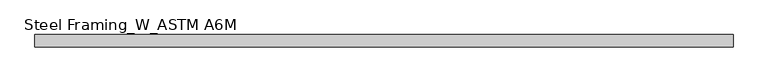
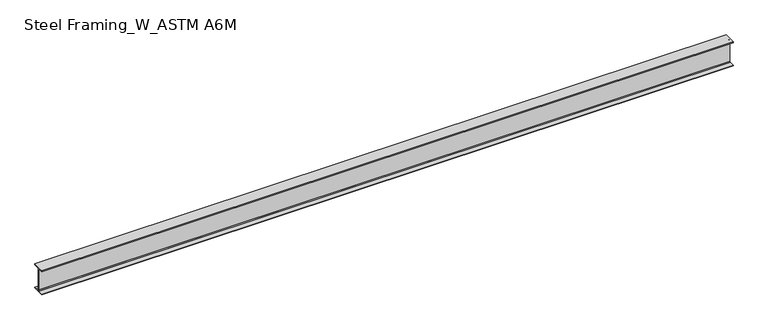
"""IFC4 building model written with IfcOpenShell, lengths in millimetres: beam geometry, Steel Framing_W_ASTM A6M : H_SB_AR_S02_W360x51_B4."""

from ifc_helpers import new_model, si_unit, point, frame, frame_2d, origin, place, context, project, spatial, polyline, circle_curve, trimmed, segment, composite_curve, outline, extrude, source, transform, mapped, element, save


def steel_framing_w_astm_a6m_aee8f6e1(model_context):
    return source(origin(), model_context, "Body", "SweptSolid", [
        extrude(outline(composite_curve([segment(polyline([(85.5, -166.4), (85.5, -178.0), (-85.5, -178.0), (-85.5, -166.4), (-13.72, -166.4)]), True, "CONTINUOUS"), segment(trimmed(circle_curve(frame_2d((-13.72, -156.3)), 10.1), [point((-13.72, -166.4))], [point((-3.62, -156.3))], True, "CARTESIAN"), True, "CONTINUOUS"), segment(polyline([(-3.62, -156.3), (-3.62, 156.3)]), True, "CONTINUOUS"), segment(trimmed(circle_curve(frame_2d((-13.72, 156.3)), 10.1), [point((-3.62, 156.3))], [point((-13.72, 166.4))], True, "CARTESIAN"), True, "CONTINUOUS"), segment(polyline([(-13.72, 166.4), (-85.5, 166.4), (-85.5, 178.0), (85.5, 178.0), (85.5, 166.4), (13.72, 166.4)]), True, "CONTINUOUS"), segment(trimmed(circle_curve(frame_2d((13.72, 156.3)), 10.1), [point((13.72, 166.4))], [point((3.62, 156.3))], True, "CARTESIAN"), True, "CONTINUOUS"), segment(polyline([(3.62, 156.3), (3.62, -156.3)]), True, "CONTINUOUS"), segment(trimmed(circle_curve(frame_2d((13.72, -156.3)), 10.1), [point((3.62, -156.3))], [point((13.72, -166.4))], True, "CARTESIAN"), True, "CONTINUOUS"), segment(polyline([(13.72, -166.4), (85.5, -166.4)]), True, "CONTINUOUS")], self_intersect=False)), frame((-4846.3, 0.0, 0.0), z_axis=(1.0, 0.0, 0.0), x_axis=(0.0, 1.0, 0.0)), (0.0, 0.0, 1.0), 9692.6),
    ])


if __name__ == "__main__":
    model = new_model("IFC4")
    model_context = context("Model", 3, world=origin())
    ifc_project = project(units=[si_unit("LENGTHUNIT", "METRE", prefix="MILLI")], contexts=[model_context])
    site = spatial("IfcSite", under=ifc_project)
    building = spatial("IfcBuilding", under=site)
    placement = place(None, origin())
    steel_framing_w_astm_a6m_shape = steel_framing_w_astm_a6m_aee8f6e1(model_context)
    element("IfcBeam", 1, ObjectType="Steel Framing_W_ASTM A6M : H_SB_AR_S02_W360x51_B4", at=placement, inside=building, context=model_context, shape_type="MappedRepresentation", body=[
        mapped(steel_framing_w_astm_a6m_shape, transform((0.0, 0.0, 0.0), x_axis=(1.0, 0.0, 0.0), y_axis=(0.0, 1.0, 0.0), z_axis=(0.0, 0.0, 1.0))),
    ])
    save(model, "model.ifc")

# Revit data of these elements
# Type "Steel Framing_W_ASTM A6M : H_SB_AR_S02_W360x51_B4"
#   Type Mark = "B4"
#   Section Name Key = "W14x34"
#   Width = 17.1 cm
#   Web Thickness = 0.724 cm
#   Web Fillet = 1.01 cm
#   Warping Constant = 287000.0 cm⁶
#   Torsional Moment of Inertia = 23.70 cm⁴
#   Section Area = 64.5 cm²
#   Plastic Modulus weak axis = 174.0 cm³
#   Plastic Modulus strong axis = 895.0 cm³
#   Perimeter = 1.36 m²/m
#   Nominal Weight = 51.00 kgf/m
#   Moment of Inertia weak axis = 970.00 cm⁴
#   Moment of Inertia strong axis = 14200.00 cm⁴
#   Height = 35.6 cm
#   Flange Thickness = 1.16 cm
#   Elastic Modulus weak axis = 113.0 cm³
#   Elastic Modulus strong axis = 796.0 cm³
#   Centroid Vertical = 17.8 cm
#   Centroid Horizontal = 8.55 cm
#   Length [instance default] = 1500 mm
#   Structural Material [instance default] = Steel, 45-345
#   Bolt Spacing = 0
#   Assembly Code = ""
# Element 1 (IfcBeam, "Steel Framing_W_ASTM A6M : H_SB_AR_S02_W360x51_B4")
#   Materials on its faces: "Steel, 45-345"
# Materials
#   "Steel, 45-345": class "Metal", colour RGB 189 187 185, transparency 0, Description = "Steel 345 MPa", Cost = 0
